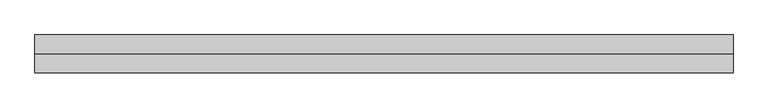
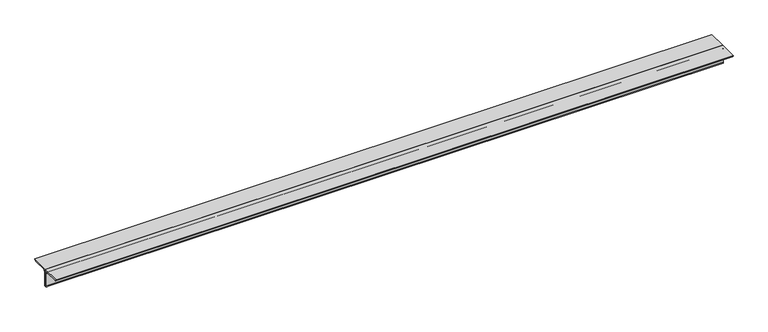
"""IFC4 building model written with IfcOpenShell, lengths in millimetres: member geometry, 0123_Steel Framing_2Ls-KSD3502 : H_SB_AR_S03_2Ls-130x130x12_HBR4."""

import ifcopenshell
import ifcopenshell.guid

model = None  # the IFC model being written
_history = None  # IfcOwnerHistory: only IFC2X3 demands one
_inside = {}  # id of a spatial element -> (the spatial element, [elements in it])
_under = {}  # id of a project, library or spatial element -> (it, [spatial elements below it])
_declared = {}  # id of a project -> (the project, [libraries it declares])
_typed = {}  # id of a type object -> (the type object, [elements of that type])
_made_of = {}  # id of a material, layer set ... -> (it, [elements and type objects made of it])


def new_model(schema):
    """Start an empty IFC model of exactly this schema.

    Asked for "IFC4X3", IfcOpenShell would pick the latest addendum, in which some entities
    have other attributes; the version numbers below select the first issue.
    IFC2X3 requires an IfcOwnerHistory on every rooted entity: one is made here for all.
    """
    global model, _history
    if schema == "IFC4X3":
        model = ifcopenshell.file(schema_version=(4, 3, 0, 0))
    else:
        model = ifcopenshell.file(schema=schema)
    _inside.clear()
    _under.clear()
    _declared.clear()
    _typed.clear()
    _made_of.clear()
    _history = None
    if model.schema == "IFC2X3":
        org = make("IfcOrganization", Name="unknown")
        user = make(
            "IfcPersonAndOrganization",
            ThePerson=make("IfcPerson", FamilyName="unknown"),
            TheOrganization=org,
        )
        app = make(
            "IfcApplication",
            ApplicationDeveloper=org,
            Version="unknown",
            ApplicationFullName="unknown",
            ApplicationIdentifier="unknown",
        )
        _history = make(
            "IfcOwnerHistory",
            OwningUser=user,
            OwningApplication=app,
            ChangeAction="ADDED",
            CreationDate=0,
        )
    return model


def make(cls, **values):
    """One entity of the class cls with the attributes given. An attribute that is None is left unset."""
    return model.create_entity(
        cls, **{name: value for name, value in values.items() if value is not None}
    )


def rooted(cls, **values):
    """An entity with a GlobalId (a new one), such as an element, a storey or a relation."""
    return make(cls, GlobalId=ifcopenshell.guid.new(), OwnerHistory=_history, **values)


def si_unit(unit_type, name, prefix=None):
    """IfcSIUnit, for example si_unit("LENGTHUNIT", "METRE", prefix="MILLI")."""
    return make("IfcSIUnit", UnitType=unit_type, Prefix=prefix, Name=name)


def assignment(units):
    """IfcUnitAssignment: the units of a project."""
    return None if units is None else make("IfcUnitAssignment", Units=units)


def point(xyz):
    """IfcCartesianPoint."""
    return None if xyz is None else make("IfcCartesianPoint", Coordinates=xyz)


def direction(xyz):
    """IfcDirection."""
    return None if xyz is None else make("IfcDirection", DirectionRatios=xyz)


def frame(location, z_axis=None, x_axis=None):
    """IfcAxis2Placement3D, a coordinate frame: its origin and axes. An axis left out is left unset."""
    return make(
        "IfcAxis2Placement3D",
        Location=point(location),
        Axis=direction(z_axis),
        RefDirection=direction(x_axis),
    )


def frame_2d(location, x_axis=None):
    """IfcAxis2Placement2D, a coordinate frame in the plane: its origin and x axis."""
    return make(
        "IfcAxis2Placement2D", Location=point(location), RefDirection=direction(x_axis)
    )


def origin():
    """The frame at (0, 0, 0) with its axes left unset."""
    return frame((0.0, 0.0, 0.0))


def place(relative_to, where):
    """IfcLocalPlacement: puts the frame where relative to a parent placement (None: the world)."""
    return make(
        "IfcLocalPlacement", PlacementRelTo=relative_to, RelativePlacement=where
    )


def context(
    kind, dimensions, precision=None, world=None, true_north=None, identifier=None
):
    """IfcGeometricRepresentationContext, for example the 3D "Model" context."""
    return make(
        "IfcGeometricRepresentationContext",
        ContextIdentifier=identifier,
        ContextType=kind,
        CoordinateSpaceDimension=dimensions,
        Precision=precision,
        WorldCoordinateSystem=world,
        TrueNorth=true_north,
    )


def project(units=None, contexts=None):
    """IfcProject with its units and contexts."""
    return rooted(
        "IfcProject",
        Name="project",
        RepresentationContexts=contexts,
        UnitsInContext=assignment(units),
    )


def spatial(cls, under=None, at=None, **own):
    """A site, building, storey or space (cls), placed at a placement, below another one or the project."""
    s = rooted(cls, ObjectPlacement=at, **own)
    if under is not None:
        _under.setdefault(under.id(), (under, []))[1].append(s)
    return s


def polyline(points):
    """IfcPolyline through the points."""
    return make("IfcPolyline", Points=[point(p) for p in points])


def circle_curve(where, radius):
    """IfcCircle in the frame where."""
    return make("IfcCircle", Position=where, Radius=radius)


def trimmed(basis, trim1, trim2, sense, master):
    """IfcTrimmedCurve: the piece of a basis curve between two trims."""
    return make(
        "IfcTrimmedCurve",
        BasisCurve=basis,
        Trim1=trim1,
        Trim2=trim2,
        SenseAgreement=sense,
        MasterRepresentation=master,
    )


def segment(curve, same_sense, transition):
    """IfcCompositeCurveSegment."""
    return make(
        "IfcCompositeCurveSegment",
        Transition=transition,
        SameSense=same_sense,
        ParentCurve=curve,
    )


def composite_curve(segments, self_intersect=None):
    """IfcCompositeCurve: segments joined end to end."""
    return make("IfcCompositeCurve", Segments=segments, SelfIntersect=self_intersect)


def outline(outer, holes=None, kind="AREA"):
    """IfcArbitraryClosedProfileDef: a profile drawn as a closed curve; with holes, ...WithVoids."""
    if holes is None:
        return make("IfcArbitraryClosedProfileDef", ProfileType=kind, OuterCurve=outer)
    return make(
        "IfcArbitraryProfileDefWithVoids",
        ProfileType=kind,
        OuterCurve=outer,
        InnerCurves=holes,
    )


def extrude(swept, where, along, depth):
    """IfcExtrudedAreaSolid: the profile swept, set in the frame where, extruded along a direction by depth."""
    return make(
        "IfcExtrudedAreaSolid",
        SweptArea=swept,
        Position=where,
        ExtrudedDirection=direction(along),
        Depth=depth,
    )


def shape(context_of_items, identifier, shape_type, items):
    """IfcShapeRepresentation: the items that make up one representation, for example the "Body"."""
    return make(
        "IfcShapeRepresentation",
        ContextOfItems=context_of_items,
        RepresentationIdentifier=identifier,
        RepresentationType=shape_type,
        Items=items,
    )


def source(mapping_origin, context_of_items, identifier, shape_type, items):
    """IfcRepresentationMap: a shape defined once, which mapped items show again and again."""
    return make(
        "IfcRepresentationMap",
        MappingOrigin=mapping_origin,
        MappedRepresentation=shape(context_of_items, identifier, shape_type, items),
    )


def transform(
    local_origin,
    x_axis=None,
    y_axis=None,
    z_axis=None,
    scale=None,
    scale2=None,
    scale3=None,
    uniform=True,
):
    """IfcCartesianTransformationOperator3D, or its non-uniform kind. x_axis, y_axis, z_axis: its Axis1, 2, 3."""
    if uniform:
        return make(
            "IfcCartesianTransformationOperator3D",
            Axis1=direction(x_axis),
            Axis2=direction(y_axis),
            LocalOrigin=point(local_origin),
            Scale=scale,
            Axis3=direction(z_axis),
        )
    return make(
        "IfcCartesianTransformationOperator3DnonUniform",
        Axis1=direction(x_axis),
        Axis2=direction(y_axis),
        LocalOrigin=point(local_origin),
        Scale=scale,
        Axis3=direction(z_axis),
        Scale2=scale2,
        Scale3=scale3,
    )


def mapped(mapping_source, mapping_target):
    """IfcMappedItem: shows the shape of a source again, moved by a transform."""
    return make(
        "IfcMappedItem", MappingSource=mapping_source, MappingTarget=mapping_target
    )


def made_of(thing, what):
    """Note that an element or type object is made of a material, layer set ...; save() writes the relation."""
    if what is not None:
        _made_of.setdefault(what.id(), (what, []))[1].append(thing)
    return thing


def element(
    cls,
    number,
    at=None,
    inside=None,
    cuts=None,
    type_object=None,
    material=None,
    context=None,
    identifier="Body",
    shape_type=None,
    held_by="IfcProductDefinitionShape",
    body=None,
    shapes=None,
    **own,
):
    """One element of the class cls, such as IfcWall. Its Tag is "e" and its number.

    at: its placement. inside: the storey or other place that contains it. cuts: it is an
    opening in that element (IfcRelVoidsElement). A single representation is given by context,
    identifier, shape_type and body (its items); several are given by shapes. held_by: the class
    of the entity that holds the representations. save() writes the other relations.
    """
    e = rooted(cls, Tag="e%d" % number, ObjectPlacement=at, **own)
    if body is not None:
        shapes = [shape(context, identifier, shape_type, body)]
    if shapes is not None:
        e.Representation = make(held_by, Representations=shapes)
    if inside is not None:
        _inside.setdefault(inside.id(), (inside, []))[1].append(e)
    if cuts is not None:
        rooted(
            "IfcRelVoidsElement", RelatingBuildingElement=cuts, RelatedOpeningElement=e
        )
    if type_object is not None:
        _typed.setdefault(type_object.id(), (type_object, []))[1].append(e)
    return made_of(e, material)


def aggregate(whole, parts):
    """IfcRelAggregates: a whole, such as a stair, and the parts it consists of."""
    return rooted("IfcRelAggregates", RelatingObject=whole, RelatedObjects=parts)


def save(model, path):
    """Write the relations noted so far, then the file.

    IfcRelAggregates (storeys below a building ...), IfcRelContainedInSpatialStructure (elements
    in a storey), IfcRelDefinesByType, IfcRelAssociatesMaterial and IfcRelDeclares: one each for
    every whole, place, type object, material and project.
    """
    for whole, parts in _under.values():
        aggregate(whole, parts)
    for where, things in _inside.values():
        rooted(
            "IfcRelContainedInSpatialStructure",
            RelatedElements=things,
            RelatingStructure=where,
        )
    for kind, things in _typed.values():
        rooted("IfcRelDefinesByType", RelatedObjects=things, RelatingType=kind)
    for what, things in _made_of.values():
        rooted("IfcRelAssociatesMaterial", RelatedObjects=things, RelatingMaterial=what)
    for by, libraries in _declared.values():
        rooted("IfcRelDeclares", RelatingContext=by, RelatedDefinitions=libraries)
    model.write(path)


def member_ef68aef1(model_context):
    return source(origin(), model_context, "Body", "SweptSolid", [
        extrude(outline(composite_curve([segment(polyline([(0.0, 36.4), (130.0, 36.4)]), True, "CONTINUOUS"), segment(trimmed(circle_curve(frame_2d((118.0, 36.4)), 12.0), [point((130.0, 36.4))], [point((118.0, 24.4))], False, "CARTESIAN"), True, "CONTINUOUS"), segment(polyline([(118.0, 24.4), (24.0, 24.4)]), True, "CONTINUOUS"), segment(trimmed(circle_curve(frame_2d((24.0, 12.4)), 12.0), [point((24.0, 24.4))], [point((12.0, 12.4))], True, "CARTESIAN"), True, "CONTINUOUS"), segment(polyline([(12.0, 12.4), (12.0, -81.6)]), True, "CONTINUOUS"), segment(trimmed(circle_curve(frame_2d((0.0, -81.6)), 12.0), [point((12.0, -81.6))], [point((0.0, -93.6))], False, "CARTESIAN"), True, "CONTINUOUS"), segment(polyline([(0.0, -93.6), (0.0, 36.4)]), True, "CONTINUOUS")], self_intersect=False)), frame((-2238.4043387, 0.0, 0.0), z_axis=(1.0, 0.0, 0.0), x_axis=(0.0, 1.0, 0.0)), (0.0, 0.0, 1.0), 4798.1465182),
        extrude(outline(composite_curve([segment(polyline([(0.0, 36.4), (0.0, -93.6)]), True, "CONTINUOUS"), segment(trimmed(circle_curve(frame_2d((0.0, -81.6)), 12.0), [point((0.0, -93.6))], [point((-12.0, -81.6))], False, "CARTESIAN"), True, "CONTINUOUS"), segment(polyline([(-12.0, -81.6), (-12.0, 12.4)]), True, "CONTINUOUS"), segment(trimmed(circle_curve(frame_2d((-24.0, 12.4)), 12.0), [point((-12.0, 12.4))], [point((-24.0, 24.4))], True, "CARTESIAN"), True, "CONTINUOUS"), segment(polyline([(-24.0, 24.4), (-118.0, 24.4)]), True, "CONTINUOUS"), segment(trimmed(circle_curve(frame_2d((-118.0, 36.4)), 12.0), [point((-118.0, 24.4))], [point((-130.0, 36.4))], False, "CARTESIAN"), True, "CONTINUOUS"), segment(polyline([(-130.0, 36.4), (0.0, 36.4)]), True, "CONTINUOUS")], self_intersect=False)), frame((-2238.4043387, 0.0, 0.0), z_axis=(1.0, 0.0, 0.0), x_axis=(0.0, 1.0, 0.0)), (0.0, 0.0, 1.0), 4798.1465182),
    ])


if __name__ == "__main__":
    model = new_model("IFC4")
    model_context = context("Model", 3, world=origin())
    ifc_project = project(units=[si_unit("LENGTHUNIT", "METRE", prefix="MILLI")], contexts=[model_context])
    site = spatial("IfcSite", under=ifc_project)
    building = spatial("IfcBuilding", under=site)
    placement = place(None, origin())
    member_shape = member_ef68aef1(model_context)
    element("IfcMember", 1, ObjectType="0123_Steel Framing_2Ls-KSD3502 : H_SB_AR_S03_2Ls-130x130x12_HBR4", at=placement, inside=building, context=model_context, shape_type="MappedRepresentation", body=[
        mapped(member_shape, transform((0.0, 0.0, 0.0), x_axis=(1.0, 0.0, 0.0), y_axis=(0.0, 1.0, 0.0), z_axis=(0.0, 0.0, 1.0))),
    ])
    save(model, "model.ifc")

# Revit data of these elements
# Type "0123_Steel Framing_2Ls-KSD3502 : H_SB_AR_S03_2Ls-130x130x12_HBR4"
#   Type Mark = "HBR4"
#   Assembly Code = "B10"
#   Legs = "SLBB"
#   W = 8.97
#   Perimeter = 1.04 m²/m
#   Nominal Weight = 46.80 kgf/m
#   Length [instance default] = 1000 mm
#   Space = 0 mm
#   b = 130 mm
#   d = 130 mm
#   t = 12 mm
#   y = 36.4 mm
#   A = 0.005952 m²
#   Structural Material [instance default] = Steel ASTM A36
# Element 1 (IfcMember, "0123_Steel Framing_2Ls-KSD3502 : H_SB_AR_S03_2Ls-130x130x12_HBR4")
#   Materials on its faces: "Steel ASTM A36"
# Materials
#   "Steel ASTM A36": class "Metal", colour RGB 199 199 199, transparency 0, Description = "Structural steel, ASTM A36 Grade B, mill finish", Cost = 0
